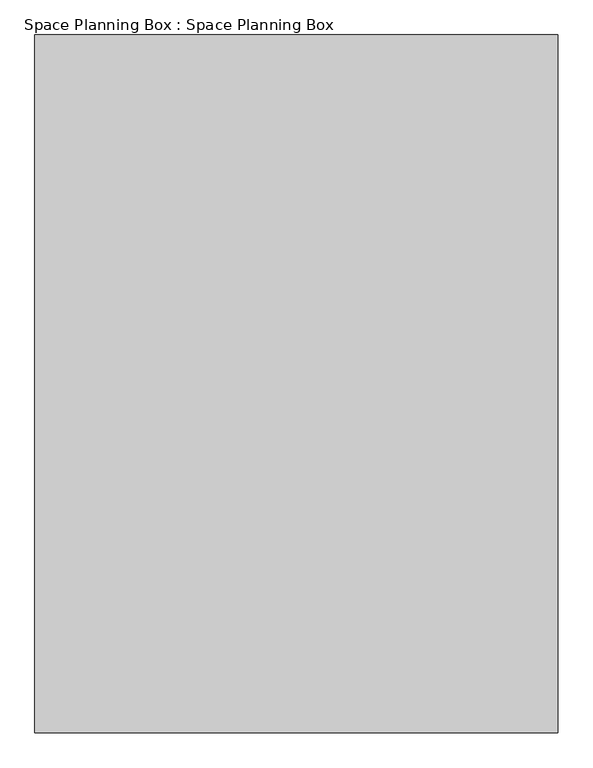
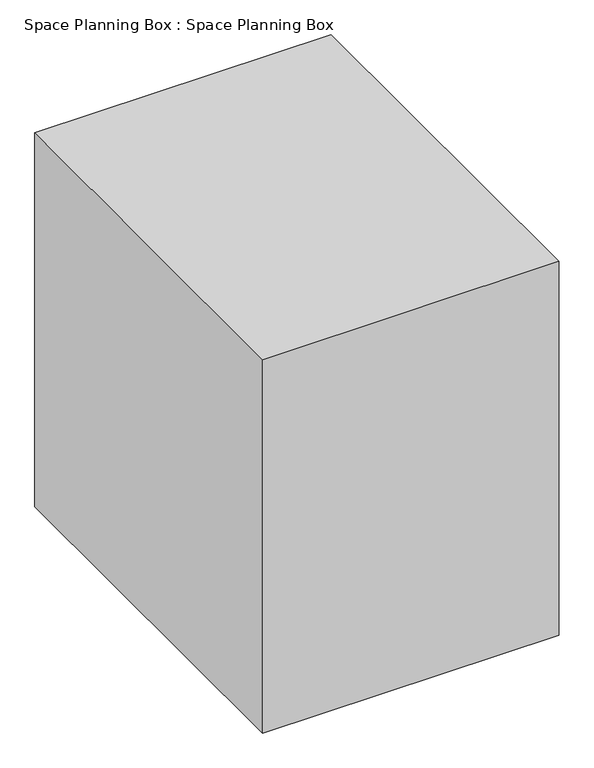
"""IFC4 building model written with IfcOpenShell, lengths in millimetres: proxy geometry, Space Planning Box : Space Planning Box."""

import ifcopenshell
import ifcopenshell.guid

model = None  # the IFC model being written
_history = None  # IfcOwnerHistory: only IFC2X3 demands one
_inside = {}  # id of a spatial element -> (the spatial element, [elements in it])
_under = {}  # id of a project, library or spatial element -> (it, [spatial elements below it])
_declared = {}  # id of a project -> (the project, [libraries it declares])
_typed = {}  # id of a type object -> (the type object, [elements of that type])
_made_of = {}  # id of a material, layer set ... -> (it, [elements and type objects made of it])


def new_model(schema):
    """Start an empty IFC model of exactly this schema.

    Asked for "IFC4X3", IfcOpenShell would pick the latest addendum, in which some entities
    have other attributes; the version numbers below select the first issue.
    IFC2X3 requires an IfcOwnerHistory on every rooted entity: one is made here for all.
    """
    global model, _history
    if schema == "IFC4X3":
        model = ifcopenshell.file(schema_version=(4, 3, 0, 0))
    else:
        model = ifcopenshell.file(schema=schema)
    _inside.clear()
    _under.clear()
    _declared.clear()
    _typed.clear()
    _made_of.clear()
    _history = None
    if model.schema == "IFC2X3":
        org = make("IfcOrganization", Name="unknown")
        user = make(
            "IfcPersonAndOrganization",
            ThePerson=make("IfcPerson", FamilyName="unknown"),
            TheOrganization=org,
        )
        app = make(
            "IfcApplication",
            ApplicationDeveloper=org,
            Version="unknown",
            ApplicationFullName="unknown",
            ApplicationIdentifier="unknown",
        )
        _history = make(
            "IfcOwnerHistory",
            OwningUser=user,
            OwningApplication=app,
            ChangeAction="ADDED",
            CreationDate=0,
        )
    return model


def make(cls, **values):
    """One entity of the class cls with the attributes given. An attribute that is None is left unset."""
    return model.create_entity(
        cls, **{name: value for name, value in values.items() if value is not None}
    )


def rooted(cls, **values):
    """An entity with a GlobalId (a new one), such as an element, a storey or a relation."""
    return make(cls, GlobalId=ifcopenshell.guid.new(), OwnerHistory=_history, **values)


def si_unit(unit_type, name, prefix=None):
    """IfcSIUnit, for example si_unit("LENGTHUNIT", "METRE", prefix="MILLI")."""
    return make("IfcSIUnit", UnitType=unit_type, Prefix=prefix, Name=name)


def assignment(units):
    """IfcUnitAssignment: the units of a project."""
    return None if units is None else make("IfcUnitAssignment", Units=units)


def point(xyz):
    """IfcCartesianPoint."""
    return None if xyz is None else make("IfcCartesianPoint", Coordinates=xyz)


def direction(xyz):
    """IfcDirection."""
    return None if xyz is None else make("IfcDirection", DirectionRatios=xyz)


def frame(location, z_axis=None, x_axis=None):
    """IfcAxis2Placement3D, a coordinate frame: its origin and axes. An axis left out is left unset."""
    return make(
        "IfcAxis2Placement3D",
        Location=point(location),
        Axis=direction(z_axis),
        RefDirection=direction(x_axis),
    )


def origin():
    """The frame at (0, 0, 0) with its axes left unset."""
    return frame((0.0, 0.0, 0.0))


def origin_with_axes():
    """The frame at (0, 0, 0) with the z axis (0, 0, 1) and the x axis (1, 0, 0) written out."""
    return frame((0.0, 0.0, 0.0), z_axis=(0.0, 0.0, 1.0), x_axis=(1.0, 0.0, 0.0))


def place(relative_to, where):
    """IfcLocalPlacement: puts the frame where relative to a parent placement (None: the world)."""
    return make(
        "IfcLocalPlacement", PlacementRelTo=relative_to, RelativePlacement=where
    )


def context(
    kind, dimensions, precision=None, world=None, true_north=None, identifier=None
):
    """IfcGeometricRepresentationContext, for example the 3D "Model" context."""
    return make(
        "IfcGeometricRepresentationContext",
        ContextIdentifier=identifier,
        ContextType=kind,
        CoordinateSpaceDimension=dimensions,
        Precision=precision,
        WorldCoordinateSystem=world,
        TrueNorth=true_north,
    )


def project(units=None, contexts=None):
    """IfcProject with its units and contexts."""
    return rooted(
        "IfcProject",
        Name="project",
        RepresentationContexts=contexts,
        UnitsInContext=assignment(units),
    )


def spatial(cls, under=None, at=None, **own):
    """A site, building, storey or space (cls), placed at a placement, below another one or the project."""
    s = rooted(cls, ObjectPlacement=at, **own)
    if under is not None:
        _under.setdefault(under.id(), (under, []))[1].append(s)
    return s


def polyline(points):
    """IfcPolyline through the points."""
    return make("IfcPolyline", Points=[point(p) for p in points])


def outline(outer, holes=None, kind="AREA"):
    """IfcArbitraryClosedProfileDef: a profile drawn as a closed curve; with holes, ...WithVoids."""
    if holes is None:
        return make("IfcArbitraryClosedProfileDef", ProfileType=kind, OuterCurve=outer)
    return make(
        "IfcArbitraryProfileDefWithVoids",
        ProfileType=kind,
        OuterCurve=outer,
        InnerCurves=holes,
    )


def extrude(swept, where, along, depth):
    """IfcExtrudedAreaSolid: the profile swept, set in the frame where, extruded along a direction by depth."""
    return make(
        "IfcExtrudedAreaSolid",
        SweptArea=swept,
        Position=where,
        ExtrudedDirection=direction(along),
        Depth=depth,
    )


def shape(context_of_items, identifier, shape_type, items):
    """IfcShapeRepresentation: the items that make up one representation, for example the "Body"."""
    return make(
        "IfcShapeRepresentation",
        ContextOfItems=context_of_items,
        RepresentationIdentifier=identifier,
        RepresentationType=shape_type,
        Items=items,
    )


def source(mapping_origin, context_of_items, identifier, shape_type, items):
    """IfcRepresentationMap: a shape defined once, which mapped items show again and again."""
    return make(
        "IfcRepresentationMap",
        MappingOrigin=mapping_origin,
        MappedRepresentation=shape(context_of_items, identifier, shape_type, items),
    )


def transform(
    local_origin,
    x_axis=None,
    y_axis=None,
    z_axis=None,
    scale=None,
    scale2=None,
    scale3=None,
    uniform=True,
):
    """IfcCartesianTransformationOperator3D, or its non-uniform kind. x_axis, y_axis, z_axis: its Axis1, 2, 3."""
    if uniform:
        return make(
            "IfcCartesianTransformationOperator3D",
            Axis1=direction(x_axis),
            Axis2=direction(y_axis),
            LocalOrigin=point(local_origin),
            Scale=scale,
            Axis3=direction(z_axis),
        )
    return make(
        "IfcCartesianTransformationOperator3DnonUniform",
        Axis1=direction(x_axis),
        Axis2=direction(y_axis),
        LocalOrigin=point(local_origin),
        Scale=scale,
        Axis3=direction(z_axis),
        Scale2=scale2,
        Scale3=scale3,
    )


def mapped(mapping_source, mapping_target):
    """IfcMappedItem: shows the shape of a source again, moved by a transform."""
    return make(
        "IfcMappedItem", MappingSource=mapping_source, MappingTarget=mapping_target
    )


def made_of(thing, what):
    """Note that an element or type object is made of a material, layer set ...; save() writes the relation."""
    if what is not None:
        _made_of.setdefault(what.id(), (what, []))[1].append(thing)
    return thing


def element(
    cls,
    number,
    at=None,
    inside=None,
    cuts=None,
    type_object=None,
    material=None,
    context=None,
    identifier="Body",
    shape_type=None,
    held_by="IfcProductDefinitionShape",
    body=None,
    shapes=None,
    **own,
):
    """One element of the class cls, such as IfcWall. Its Tag is "e" and its number.

    at: its placement. inside: the storey or other place that contains it. cuts: it is an
    opening in that element (IfcRelVoidsElement). A single representation is given by context,
    identifier, shape_type and body (its items); several are given by shapes. held_by: the class
    of the entity that holds the representations. save() writes the other relations.
    """
    e = rooted(cls, Tag="e%d" % number, ObjectPlacement=at, **own)
    if body is not None:
        shapes = [shape(context, identifier, shape_type, body)]
    if shapes is not None:
        e.Representation = make(held_by, Representations=shapes)
    if inside is not None:
        _inside.setdefault(inside.id(), (inside, []))[1].append(e)
    if cuts is not None:
        rooted(
            "IfcRelVoidsElement", RelatingBuildingElement=cuts, RelatedOpeningElement=e
        )
    if type_object is not None:
        _typed.setdefault(type_object.id(), (type_object, []))[1].append(e)
    return made_of(e, material)


def aggregate(whole, parts):
    """IfcRelAggregates: a whole, such as a stair, and the parts it consists of."""
    return rooted("IfcRelAggregates", RelatingObject=whole, RelatedObjects=parts)


def save(model, path):
    """Write the relations noted so far, then the file.

    IfcRelAggregates (storeys below a building ...), IfcRelContainedInSpatialStructure (elements
    in a storey), IfcRelDefinesByType, IfcRelAssociatesMaterial and IfcRelDeclares: one each for
    every whole, place, type object, material and project.
    """
    for whole, parts in _under.values():
        aggregate(whole, parts)
    for where, things in _inside.values():
        rooted(
            "IfcRelContainedInSpatialStructure",
            RelatedElements=things,
            RelatingStructure=where,
        )
    for kind, things in _typed.values():
        rooted("IfcRelDefinesByType", RelatedObjects=things, RelatingType=kind)
    for what, things in _made_of.values():
        rooted("IfcRelAssociatesMaterial", RelatedObjects=things, RelatingMaterial=what)
    for by, libraries in _declared.values():
        rooted("IfcRelDeclares", RelatingContext=by, RelatedDefinitions=libraries)
    model.write(path)


def space_planning_box_space_planning_box_8af91fed(model_context):
    return source(origin(), model_context, "Body", "SweptSolid", [
        extrude(outline(polyline([(2250.0, 3000.0), (2250.0, -3000.0), (-2250.0, -3000.0), (-2250.0, 3000.0), (2250.0, 3000.0)])), origin_with_axes(), (0.0, 0.0, 1.0), 6000.0),
    ])


if __name__ == "__main__":
    model = new_model("IFC4")
    model_context = context("Model", 3, world=origin())
    ifc_project = project(units=[si_unit("LENGTHUNIT", "METRE", prefix="MILLI")], contexts=[model_context])
    site = spatial("IfcSite", under=ifc_project)
    building = spatial("IfcBuilding", under=site)
    placement = place(None, origin())
    space_planning_box_space_planning_box_shape = space_planning_box_space_planning_box_8af91fed(model_context)
    element("IfcBuildingElementProxy", 1, Name="Space Planning Box : Space Planning Box", ObjectType="Space Planning Box : Space Planning Box", at=placement, inside=building, context=model_context, shape_type="MappedRepresentation", body=[
        mapped(space_planning_box_space_planning_box_shape, transform((0.0, 0.0, 0.0), x_axis=(1.0, 0.0, 0.0), y_axis=(0.0, 1.0, 0.0), z_axis=(0.0, 0.0, 1.0))),
    ])
    save(model, "model.ifc")

# Revit data of these elements
# Type "Space Planning Box : Space Planning Box"
#   Type Comments = "..."
#   Room Name [instance default] = "?"
#   Assembly Code = "..."
#   Width [instance default] = 1524 mm
#   Program Area [instance default] = 0 m²
#   Length [instance default] = 1524 mm
#   Height [instance default] = 1524 mm
#   Area [instance default] = 2.32258 m²
#   Fill Color [instance default] = Cyan
#   Default Elevation = 0
# Element 1 (IfcBuildingElementProxy, "Space Planning Box : Space Planning Box")
#   Room Name = "Shift Office Room"
#   Width = 4500 mm
#   Program Area = 43.2 m²
#   Length = 6000 mm
#   Height = 6000 mm
#   Area = 27 m²
#   Fill Color = Lavender
#   Materials on its faces: "Lavender"
# Materials
#   "Cyan": class "Generic", colour RGB 0 255 255, transparency 0.2, Cost = 0
#   "Lavender": class "Generic", colour RGB 186 85 211, transparency 0.2, Cost = 0
